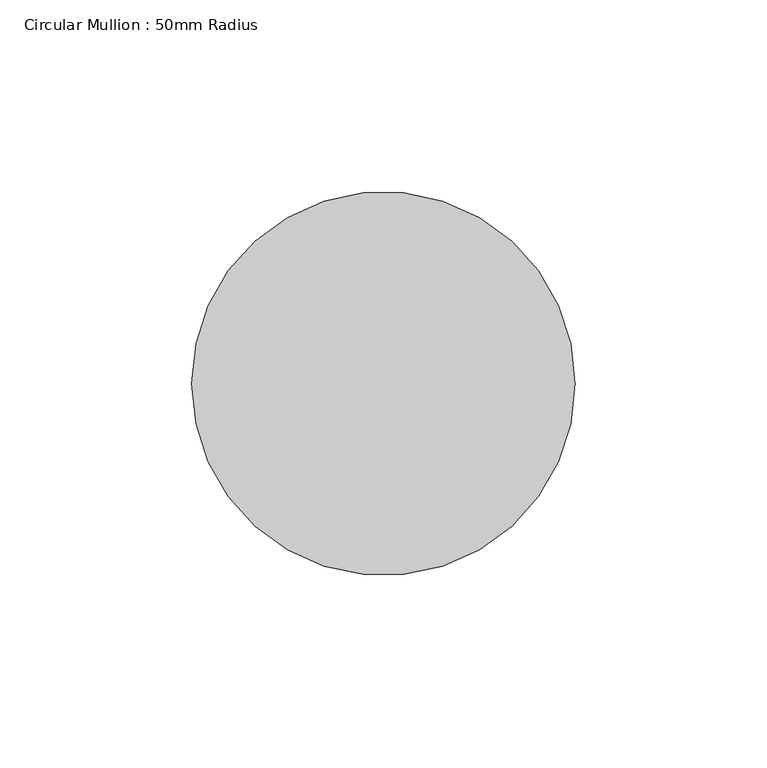
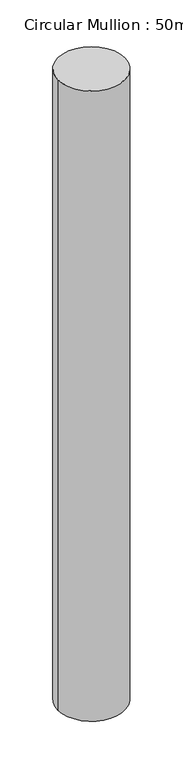
"""IFC4 building model written with IfcOpenShell, lengths in millimetres: member geometry, Circular Mullion : 50mm Radius."""

from ifc_helpers import new_model, si_unit, point, frame, origin, origin_2d, place, context, project, spatial, circle_curve, trimmed, segment, composite_curve, outline, extrude, source, transform, mapped, element, save


def circular_mullion_50mm_radius_de71cea4(model_context):
    return source(origin(), model_context, "Body", "SweptSolid", [
        extrude(outline(composite_curve([segment(trimmed(circle_curve(origin_2d(), 50.0), [point((50.0, 0.0))], [point((-50.0, 0.0))], False, "CARTESIAN"), True, "CONTINUOUS"), segment(trimmed(circle_curve(origin_2d(), 50.0), [point((-50.0, 0.0))], [point((50.0, 0.0))], False, "CARTESIAN"), True, "CONTINUOUS")], self_intersect=False)), frame((0.0, 0.0, -996.3030919), z_axis=(0.0, 0.0, 1.0), x_axis=(1.0, 0.0, 0.0)), (0.0, 0.0, 1.0), 996.3030919),
    ])


if __name__ == "__main__":
    model = new_model("IFC4")
    model_context = context("Model", 3, world=origin())
    ifc_project = project(units=[si_unit("LENGTHUNIT", "METRE", prefix="MILLI")], contexts=[model_context])
    site = spatial("IfcSite", under=ifc_project)
    building = spatial("IfcBuilding", under=site)
    placement = place(None, origin())
    circular_mullion_50mm_radius_shape = circular_mullion_50mm_radius_de71cea4(model_context)
    element("IfcMember", 1, ObjectType="Circular Mullion : 50mm Radius", at=placement, inside=building, context=model_context, shape_type="MappedRepresentation", body=[
        mapped(circular_mullion_50mm_radius_shape, transform((0.0, 0.0, 0.0), x_axis=(1.0, 0.0, 0.0), y_axis=(0.0, 1.0, 0.0), z_axis=(0.0, 0.0, 1.0))),
    ])
    save(model, "model.ifc")

# Revit data of these elements
# Type "Circular Mullion : 50mm Radius"
#   built-in parameter 1007350 = 0.164042 (stored number, unit not read)
# Element 1 (IfcMember, "Circular Mullion : 50mm Radius")
#   Materials on its faces: "Aluminium"
# Materials
#   "Aluminium": class "Metal", colour RGB 247 247 247, transparency 0, Description = "Aluminium 6061", Cost = 0
